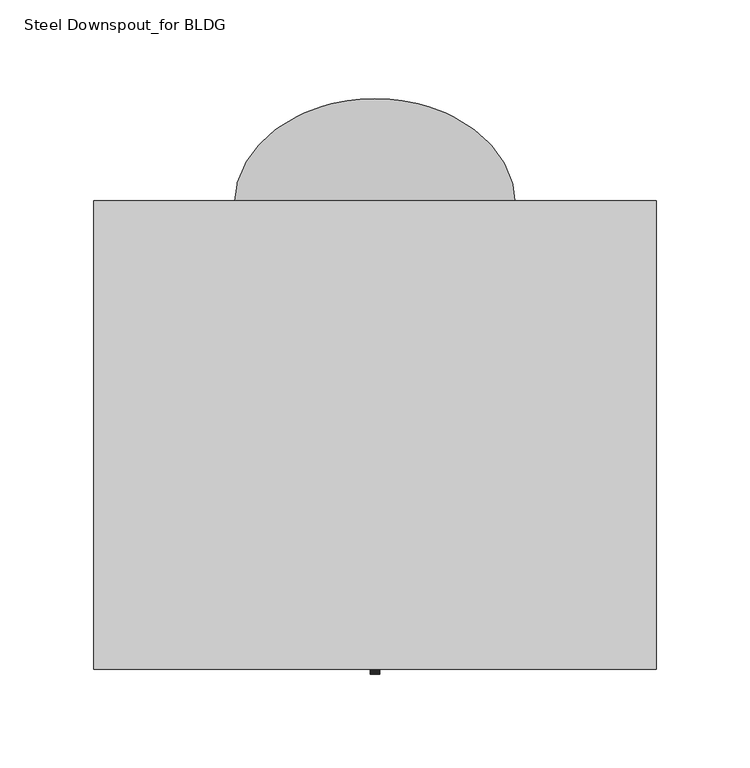
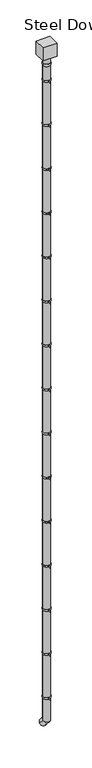
"""IFC4 building model written with IfcOpenShell, lengths in millimetres: proxy geometry, Steel Downspout_for BLDG : H_GM_AR_B07_Steel Downspout_D150."""

from ifc_helpers import new_model, si_unit, point, frame, origin, origin_with_axes, origin_2d, place, context, project, spatial, polyline, circle_curve, ellipse_curve, trimmed, segment, composite_curve, outline, extrude, source, transform, mapped, element, save
from ifc_brep_helpers import plane_surface, cylinder_surface, revolved_surface, advanced_brep


def steel_downspout_for_bldg_2e53916e(model_context):
    return source(origin(), model_context, "Body", "SolidModel", [
        extrude(outline(polyline([(2.5, -125.0), (-2.5, -125.0), (-2.5, -50.0), (2.5, -50.0), (2.5, -125.0)])), frame((0.0, 0.0, -556.0), z_axis=(0.0, 0.0, 1.0), x_axis=(1.0, 0.0, 0.0)), (0.0, 0.0, 1.0), 32.0),
        extrude(outline(composite_curve([segment(trimmed(circle_curve(origin_2d(), 80.0), [point((0.0, 80.0))], [point((0.0, -80.0))], False, "CARTESIAN"), True, "CONTINUOUS"), segment(trimmed(circle_curve(origin_2d(), 80.0), [point((0.0, -80.0))], [point((0.0, 80.0))], False, "CARTESIAN"), True, "CONTINUOUS")], self_intersect=False), holes=[composite_curve([segment(trimmed(circle_curve(origin_2d(), 75.0), [point((0.0, 75.0))], [point((0.0, -75.0))], True, "CARTESIAN"), True, "CONTINUOUS"), segment(trimmed(circle_curve(origin_2d(), 75.0), [point((0.0, -75.0))], [point((0.0, 75.0))], True, "CARTESIAN"), True, "CONTINUOUS")], self_intersect=False)]), frame((0.0, 0.0, -556.0), z_axis=(0.0, 0.0, 1.0), x_axis=(1.0, 0.0, 0.0)), (0.0, 0.0, 1.0), 32.0),
        extrude(outline(polyline([(2.5, -125.0), (-2.5, -125.0), (-2.5, -50.0), (2.5, -50.0), (2.5, -125.0)])), frame((0.0, 0.0, -1556.0), z_axis=(0.0, 0.0, 1.0), x_axis=(1.0, 0.0, 0.0)), (0.0, 0.0, 1.0), 32.0),
        extrude(outline(composite_curve([segment(trimmed(circle_curve(origin_2d(), 80.0), [point((0.0, 80.0))], [point((0.0, -80.0))], False, "CARTESIAN"), True, "CONTINUOUS"), segment(trimmed(circle_curve(origin_2d(), 80.0), [point((0.0, -80.0))], [point((0.0, 80.0))], False, "CARTESIAN"), True, "CONTINUOUS")], self_intersect=False), holes=[composite_curve([segment(trimmed(circle_curve(origin_2d(), 75.0), [point((0.0, 75.0))], [point((0.0, -75.0))], True, "CARTESIAN"), True, "CONTINUOUS"), segment(trimmed(circle_curve(origin_2d(), 75.0), [point((0.0, -75.0))], [point((0.0, 75.0))], True, "CARTESIAN"), True, "CONTINUOUS")], self_intersect=False)]), frame((0.0, 0.0, -1556.0), z_axis=(0.0, 0.0, 1.0), x_axis=(1.0, 0.0, 0.0)), (0.0, 0.0, 1.0), 32.0),
        extrude(outline(polyline([(2.5, -125.0), (-2.5, -125.0), (-2.5, -50.0), (2.5, -50.0), (2.5, -125.0)])), frame((0.0, 0.0, -2556.0), z_axis=(0.0, 0.0, 1.0), x_axis=(1.0, 0.0, 0.0)), (0.0, 0.0, 1.0), 32.0),
        extrude(outline(composite_curve([segment(trimmed(circle_curve(origin_2d(), 80.0), [point((0.0, 80.0))], [point((0.0, -80.0))], False, "CARTESIAN"), True, "CONTINUOUS"), segment(trimmed(circle_curve(origin_2d(), 80.0), [point((0.0, -80.0))], [point((0.0, 80.0))], False, "CARTESIAN"), True, "CONTINUOUS")], self_intersect=False), holes=[composite_curve([segment(trimmed(circle_curve(origin_2d(), 75.0), [point((0.0, 75.0))], [point((0.0, -75.0))], True, "CARTESIAN"), True, "CONTINUOUS"), segment(trimmed(circle_curve(origin_2d(), 75.0), [point((0.0, -75.0))], [point((0.0, 75.0))], True, "CARTESIAN"), True, "CONTINUOUS")], self_intersect=False)]), frame((0.0, 0.0, -2556.0), z_axis=(0.0, 0.0, 1.0), x_axis=(1.0, 0.0, 0.0)), (0.0, 0.0, 1.0), 32.0),
        extrude(outline(polyline([(2.5, -125.0), (-2.5, -125.0), (-2.5, -50.0), (2.5, -50.0), (2.5, -125.0)])), frame((0.0, 0.0, -3556.0), z_axis=(0.0, 0.0, 1.0), x_axis=(1.0, 0.0, 0.0)), (0.0, 0.0, 1.0), 32.0),
        extrude(outline(composite_curve([segment(trimmed(circle_curve(origin_2d(), 80.0), [point((0.0, 80.0))], [point((0.0, -80.0))], False, "CARTESIAN"), True, "CONTINUOUS"), segment(trimmed(circle_curve(origin_2d(), 80.0), [point((0.0, -80.0))], [point((0.0, 80.0))], False, "CARTESIAN"), True, "CONTINUOUS")], self_intersect=False), holes=[composite_curve([segment(trimmed(circle_curve(origin_2d(), 75.0), [point((0.0, 75.0))], [point((0.0, -75.0))], True, "CARTESIAN"), True, "CONTINUOUS"), segment(trimmed(circle_curve(origin_2d(), 75.0), [point((0.0, -75.0))], [point((0.0, 75.0))], True, "CARTESIAN"), True, "CONTINUOUS")], self_intersect=False)]), frame((0.0, 0.0, -3556.0), z_axis=(0.0, 0.0, 1.0), x_axis=(1.0, 0.0, 0.0)), (0.0, 0.0, 1.0), 32.0),
        extrude(outline(polyline([(2.5, -125.0), (-2.5, -125.0), (-2.5, -50.0), (2.5, -50.0), (2.5, -125.0)])), frame((0.0, 0.0, -4556.0), z_axis=(0.0, 0.0, 1.0), x_axis=(1.0, 0.0, 0.0)), (0.0, 0.0, 1.0), 32.0),
        extrude(outline(composite_curve([segment(trimmed(circle_curve(origin_2d(), 80.0), [point((0.0, 80.0))], [point((0.0, -80.0))], False, "CARTESIAN"), True, "CONTINUOUS"), segment(trimmed(circle_curve(origin_2d(), 80.0), [point((0.0, -80.0))], [point((0.0, 80.0))], False, "CARTESIAN"), True, "CONTINUOUS")], self_intersect=False), holes=[composite_curve([segment(trimmed(circle_curve(origin_2d(), 75.0), [point((0.0, 75.0))], [point((0.0, -75.0))], True, "CARTESIAN"), True, "CONTINUOUS"), segment(trimmed(circle_curve(origin_2d(), 75.0), [point((0.0, -75.0))], [point((0.0, 75.0))], True, "CARTESIAN"), True, "CONTINUOUS")], self_intersect=False)]), frame((0.0, 0.0, -4556.0), z_axis=(0.0, 0.0, 1.0), x_axis=(1.0, 0.0, 0.0)), (0.0, 0.0, 1.0), 32.0),
        extrude(outline(polyline([(2.5, -125.0), (-2.5, -125.0), (-2.5, -50.0), (2.5, -50.0), (2.5, -125.0)])), frame((0.0, 0.0, -5556.0), z_axis=(0.0, 0.0, 1.0), x_axis=(1.0, 0.0, 0.0)), (0.0, 0.0, 1.0), 32.0),
        extrude(outline(composite_curve([segment(trimmed(circle_curve(origin_2d(), 80.0), [point((0.0, 80.0))], [point((0.0, -80.0))], False, "CARTESIAN"), True, "CONTINUOUS"), segment(trimmed(circle_curve(origin_2d(), 80.0), [point((0.0, -80.0))], [point((0.0, 80.0))], False, "CARTESIAN"), True, "CONTINUOUS")], self_intersect=False), holes=[composite_curve([segment(trimmed(circle_curve(origin_2d(), 75.0), [point((0.0, 75.0))], [point((0.0, -75.0))], True, "CARTESIAN"), True, "CONTINUOUS"), segment(trimmed(circle_curve(origin_2d(), 75.0), [point((0.0, -75.0))], [point((0.0, 75.0))], True, "CARTESIAN"), True, "CONTINUOUS")], self_intersect=False)]), frame((0.0, 0.0, -5556.0), z_axis=(0.0, 0.0, 1.0), x_axis=(1.0, 0.0, 0.0)), (0.0, 0.0, 1.0), 32.0),
        extrude(outline(polyline([(2.5, -125.0), (-2.5, -125.0), (-2.5, -50.0), (2.5, -50.0), (2.5, -125.0)])), frame((0.0, 0.0, -6556.0), z_axis=(0.0, 0.0, 1.0), x_axis=(1.0, 0.0, 0.0)), (0.0, 0.0, 1.0), 32.0),
        extrude(outline(composite_curve([segment(trimmed(circle_curve(origin_2d(), 80.0), [point((0.0, 80.0))], [point((0.0, -80.0))], False, "CARTESIAN"), True, "CONTINUOUS"), segment(trimmed(circle_curve(origin_2d(), 80.0), [point((0.0, -80.0))], [point((0.0, 80.0))], False, "CARTESIAN"), True, "CONTINUOUS")], self_intersect=False), holes=[composite_curve([segment(trimmed(circle_curve(origin_2d(), 75.0), [point((0.0, 75.0))], [point((0.0, -75.0))], True, "CARTESIAN"), True, "CONTINUOUS"), segment(trimmed(circle_curve(origin_2d(), 75.0), [point((0.0, -75.0))], [point((0.0, 75.0))], True, "CARTESIAN"), True, "CONTINUOUS")], self_intersect=False)]), frame((0.0, 0.0, -6556.0), z_axis=(0.0, 0.0, 1.0), x_axis=(1.0, 0.0, 0.0)), (0.0, 0.0, 1.0), 32.0),
        extrude(outline(polyline([(2.5, -125.0), (-2.5, -125.0), (-2.5, -50.0), (2.5, -50.0), (2.5, -125.0)])), frame((0.0, 0.0, -7556.0), z_axis=(0.0, 0.0, 1.0), x_axis=(1.0, 0.0, 0.0)), (0.0, 0.0, 1.0), 32.0),
        extrude(outline(composite_curve([segment(trimmed(circle_curve(origin_2d(), 80.0), [point((0.0, 80.0))], [point((0.0, -80.0))], False, "CARTESIAN"), True, "CONTINUOUS"), segment(trimmed(circle_curve(origin_2d(), 80.0), [point((0.0, -80.0))], [point((0.0, 80.0))], False, "CARTESIAN"), True, "CONTINUOUS")], self_intersect=False), holes=[composite_curve([segment(trimmed(circle_curve(origin_2d(), 75.0), [point((0.0, 75.0))], [point((0.0, -75.0))], True, "CARTESIAN"), True, "CONTINUOUS"), segment(trimmed(circle_curve(origin_2d(), 75.0), [point((0.0, -75.0))], [point((0.0, 75.0))], True, "CARTESIAN"), True, "CONTINUOUS")], self_intersect=False)]), frame((0.0, 0.0, -7556.0), z_axis=(0.0, 0.0, 1.0), x_axis=(1.0, 0.0, 0.0)), (0.0, 0.0, 1.0), 32.0),
        extrude(outline(polyline([(2.5, -125.0), (-2.5, -125.0), (-2.5, -50.0), (2.5, -50.0), (2.5, -125.0)])), frame((0.0, 0.0, -8556.0), z_axis=(0.0, 0.0, 1.0), x_axis=(1.0, 0.0, 0.0)), (0.0, 0.0, 1.0), 32.0),
        extrude(outline(composite_curve([segment(trimmed(circle_curve(origin_2d(), 80.0), [point((0.0, 80.0))], [point((0.0, -80.0))], False, "CARTESIAN"), True, "CONTINUOUS"), segment(trimmed(circle_curve(origin_2d(), 80.0), [point((0.0, -80.0))], [point((0.0, 80.0))], False, "CARTESIAN"), True, "CONTINUOUS")], self_intersect=False), holes=[composite_curve([segment(trimmed(circle_curve(origin_2d(), 75.0), [point((0.0, 75.0))], [point((0.0, -75.0))], True, "CARTESIAN"), True, "CONTINUOUS"), segment(trimmed(circle_curve(origin_2d(), 75.0), [point((0.0, -75.0))], [point((0.0, 75.0))], True, "CARTESIAN"), True, "CONTINUOUS")], self_intersect=False)]), frame((0.0, 0.0, -8556.0), z_axis=(0.0, 0.0, 1.0), x_axis=(1.0, 0.0, 0.0)), (0.0, 0.0, 1.0), 32.0),
        extrude(outline(polyline([(2.5, -125.0), (-2.5, -125.0), (-2.5, -50.0), (2.5, -50.0), (2.5, -125.0)])), frame((0.0, 0.0, -9556.0), z_axis=(0.0, 0.0, 1.0), x_axis=(1.0, 0.0, 0.0)), (0.0, 0.0, 1.0), 32.0),
        extrude(outline(composite_curve([segment(trimmed(circle_curve(origin_2d(), 80.0), [point((0.0, 80.0))], [point((0.0, -80.0))], False, "CARTESIAN"), True, "CONTINUOUS"), segment(trimmed(circle_curve(origin_2d(), 80.0), [point((0.0, -80.0))], [point((0.0, 80.0))], False, "CARTESIAN"), True, "CONTINUOUS")], self_intersect=False), holes=[composite_curve([segment(trimmed(circle_curve(origin_2d(), 75.0), [point((0.0, 75.0))], [point((0.0, -75.0))], True, "CARTESIAN"), True, "CONTINUOUS"), segment(trimmed(circle_curve(origin_2d(), 75.0), [point((0.0, -75.0))], [point((0.0, 75.0))], True, "CARTESIAN"), True, "CONTINUOUS")], self_intersect=False)]), frame((0.0, 0.0, -9556.0), z_axis=(0.0, 0.0, 1.0), x_axis=(1.0, 0.0, 0.0)), (0.0, 0.0, 1.0), 32.0),
        extrude(outline(polyline([(2.5, -125.0), (-2.5, -125.0), (-2.5, -50.0), (2.5, -50.0), (2.5, -125.0)])), frame((0.0, 0.0, -10556.0), z_axis=(0.0, 0.0, 1.0), x_axis=(1.0, 0.0, 0.0)), (0.0, 0.0, 1.0), 32.0),
        extrude(outline(composite_curve([segment(trimmed(circle_curve(origin_2d(), 80.0), [point((0.0, 80.0))], [point((0.0, -80.0))], False, "CARTESIAN"), True, "CONTINUOUS"), segment(trimmed(circle_curve(origin_2d(), 80.0), [point((0.0, -80.0))], [point((0.0, 80.0))], False, "CARTESIAN"), True, "CONTINUOUS")], self_intersect=False), holes=[composite_curve([segment(trimmed(circle_curve(origin_2d(), 75.0), [point((0.0, 75.0))], [point((0.0, -75.0))], True, "CARTESIAN"), True, "CONTINUOUS"), segment(trimmed(circle_curve(origin_2d(), 75.0), [point((0.0, -75.0))], [point((0.0, 75.0))], True, "CARTESIAN"), True, "CONTINUOUS")], self_intersect=False)]), frame((0.0, 0.0, -10556.0), z_axis=(0.0, 0.0, 1.0), x_axis=(1.0, 0.0, 0.0)), (0.0, 0.0, 1.0), 32.0),
        extrude(outline(polyline([(2.5, -125.0), (-2.5, -125.0), (-2.5, -50.0), (2.5, -50.0), (2.5, -125.0)])), frame((0.0, 0.0, -11556.0), z_axis=(0.0, 0.0, 1.0), x_axis=(1.0, 0.0, 0.0)), (0.0, 0.0, 1.0), 32.0),
        extrude(outline(composite_curve([segment(trimmed(circle_curve(origin_2d(), 80.0), [point((0.0, 80.0))], [point((0.0, -80.0))], False, "CARTESIAN"), True, "CONTINUOUS"), segment(trimmed(circle_curve(origin_2d(), 80.0), [point((0.0, -80.0))], [point((0.0, 80.0))], False, "CARTESIAN"), True, "CONTINUOUS")], self_intersect=False), holes=[composite_curve([segment(trimmed(circle_curve(origin_2d(), 75.0), [point((0.0, 75.0))], [point((0.0, -75.0))], True, "CARTESIAN"), True, "CONTINUOUS"), segment(trimmed(circle_curve(origin_2d(), 75.0), [point((0.0, -75.0))], [point((0.0, 75.0))], True, "CARTESIAN"), True, "CONTINUOUS")], self_intersect=False)]), frame((0.0, 0.0, -11556.0), z_axis=(0.0, 0.0, 1.0), x_axis=(1.0, 0.0, 0.0)), (0.0, 0.0, 1.0), 32.0),
        extrude(outline(polyline([(2.5, -125.0), (-2.5, -125.0), (-2.5, -50.0), (2.5, -50.0), (2.5, -125.0)])), frame((0.0, 0.0, -12556.0), z_axis=(0.0, 0.0, 1.0), x_axis=(1.0, 0.0, 0.0)), (0.0, 0.0, 1.0), 32.0),
        extrude(outline(composite_curve([segment(trimmed(circle_curve(origin_2d(), 80.0), [point((0.0, 80.0))], [point((0.0, -80.0))], False, "CARTESIAN"), True, "CONTINUOUS"), segment(trimmed(circle_curve(origin_2d(), 80.0), [point((0.0, -80.0))], [point((0.0, 80.0))], False, "CARTESIAN"), True, "CONTINUOUS")], self_intersect=False), holes=[composite_curve([segment(trimmed(circle_curve(origin_2d(), 75.0), [point((0.0, 75.0))], [point((0.0, -75.0))], True, "CARTESIAN"), True, "CONTINUOUS"), segment(trimmed(circle_curve(origin_2d(), 75.0), [point((0.0, -75.0))], [point((0.0, 75.0))], True, "CARTESIAN"), True, "CONTINUOUS")], self_intersect=False)]), frame((0.0, 0.0, -12556.0), z_axis=(0.0, 0.0, 1.0), x_axis=(1.0, 0.0, 0.0)), (0.0, 0.0, 1.0), 32.0),
        extrude(outline(polyline([(2.5, -125.0), (-2.5, -125.0), (-2.5, -50.0), (2.5, -50.0), (2.5, -125.0)])), frame((0.0, 0.0, -13556.0), z_axis=(0.0, 0.0, 1.0), x_axis=(1.0, 0.0, 0.0)), (0.0, 0.0, 1.0), 32.0),
        extrude(outline(composite_curve([segment(trimmed(circle_curve(origin_2d(), 80.0), [point((0.0, 80.0))], [point((0.0, -80.0))], False, "CARTESIAN"), True, "CONTINUOUS"), segment(trimmed(circle_curve(origin_2d(), 80.0), [point((0.0, -80.0))], [point((0.0, 80.0))], False, "CARTESIAN"), True, "CONTINUOUS")], self_intersect=False), holes=[composite_curve([segment(trimmed(circle_curve(origin_2d(), 75.0), [point((0.0, 75.0))], [point((0.0, -75.0))], True, "CARTESIAN"), True, "CONTINUOUS"), segment(trimmed(circle_curve(origin_2d(), 75.0), [point((0.0, -75.0))], [point((0.0, 75.0))], True, "CARTESIAN"), True, "CONTINUOUS")], self_intersect=False)]), frame((0.0, 0.0, -13556.0), z_axis=(0.0, 0.0, 1.0), x_axis=(1.0, 0.0, 0.0)), (0.0, 0.0, 1.0), 32.0),
        advanced_brep(
        [(-75.0, 0.0, -200.0), (75.0, 0.0, -200.0), (-65.0, 0.0, -200.0), (65.0, 0.0, -200.0), (-65.0, 0.0, -15056.0), (65.0, 0.0, -15056.0), (-75.0, 0.0, -15056.0), (75.0, 0.0, -15056.0), (-75.0, 125.386264, -15200.2403969), (75.0, 125.386264, -15200.2403969), (-65.0, 125.386264, -15200.2403969), (65.0, 125.386264, -15200.2403969)],
        [
            (0, 1, circle_curve(frame((0.0, 0.0, -200.0), z_axis=(0.0, 0.0, 1.0), x_axis=(1.0, 0.0, 0.0)), 75.0)),
            (1, 0, circle_curve(frame((0.0, 0.0, -200.0), z_axis=(0.0, 0.0, 1.0), x_axis=(1.0, 0.0, 0.0)), 75.0)),
            (2, 3, circle_curve(frame((0.0, 0.0, -200.0), z_axis=(0.0, 0.0, -1.0), x_axis=(1.0, 0.0, 0.0)), 65.0)),
            (3, 2, circle_curve(frame((0.0, 0.0, -200.0), z_axis=(0.0, 0.0, -1.0), x_axis=(1.0, 0.0, 0.0)), 65.0)),
            (2, 4),
            (4, 5, ellipse_curve(frame((0.0, 0.0, -15056.0), z_axis=(0.0, 0.3502073812593857, -0.9366721892484282), x_axis=(0.0, -0.9366721892484282, -0.35020738125938544)), 69.3946086, 65.0)),
            (5, 3),
            (5, 4, ellipse_curve(frame((0.0, 0.0, -15056.0), z_axis=(0.0, 0.3502073812593857, -0.9366721892484282), x_axis=(0.0, -0.9366721892484282, -0.35020738125938544)), 69.3946086, 65.0)),
            (0, 6),
            (6, 7, ellipse_curve(frame((0.0, 0.0, -15056.0), z_axis=(0.0, -0.3502073812593857, 0.9366721892484282), x_axis=(0.0, 0.9366721892484282, 0.35020738125938544)), 80.0707023, 75.0)),
            (7, 1),
            (7, 6, ellipse_curve(frame((0.0, 0.0, -15056.0), z_axis=(0.0, -0.3502073812593857, 0.9366721892484282), x_axis=(0.0, 0.9366721892484282, 0.35020738125938544)), 80.0707023, 75.0)),
            (8, 9, circle_curve(frame((0.0, 125.386264, -15200.2403969), z_axis=(0.0, 0.6560590289903756, -0.7547095802228865), x_axis=(1.0, 0.0, 0.0)), 75.0)),
            (9, 8, circle_curve(frame((0.0, 125.386264, -15200.2403969), z_axis=(0.0, 0.6560590289903756, -0.7547095802228865), x_axis=(1.0, 0.0, 0.0)), 75.0)),
            (10, 11, circle_curve(frame((0.0, 125.386264, -15200.2403969), z_axis=(0.0, -0.6560590289903756, 0.7547095802228865), x_axis=(1.0, 0.0, 0.0)), 65.0)),
            (11, 10, circle_curve(frame((0.0, 125.386264, -15200.2403969), z_axis=(0.0, -0.6560590289903756, 0.7547095802228865), x_axis=(1.0, 0.0, 0.0)), 65.0)),
            (4, 10),
            (11, 5),
            (6, 8),
            (9, 7),
        ],
        [
            plane_surface(frame((0.0, 0.0, -200.0), z_axis=(0.0, 0.0, 1.0), x_axis=(1.0, 0.0, 0.0))),
            revolved_surface(polyline([(65.0, 0.0, -15080.302504151327), (65.0, 0.0, -200.0)]), (0.0, 0.0, -200.0), (0.0, 0.0, -1.0)),
            cylinder_surface(frame((0.0, 0.0, -200.0), z_axis=(0.0, 0.0, 1.0), x_axis=(1.0, 0.0, 0.0)), 75.0),
            plane_surface(frame((0.0, 125.386264, -15200.2403969), z_axis=(0.0, 0.6560590289903756, -0.7547095802228865), x_axis=(1.0, 0.0, 0.0))),
            revolved_surface(polyline([(65.0, 125.38626404697672, -15200.240396859164), (65.0, -15.94387727555355, -15037.658667293588)]), (0.0, 0.0, -15056.0), (0.0, 0.6560590289903756, -0.7547095802228865)),
            cylinder_surface(frame((0.0, 0.0, -15056.0), z_axis=(0.0, -0.6560590289903756, 0.7547095802228865), x_axis=(1.0, 0.0, 0.0)), 75.0),
        ],
        [
            (0, [[1, 2], [3, 4]]),
            (1, [[-3, 5, 6, 7]]),
            (1, [[-4, -7, 8, -5]]),
            (2, [[-1, 9, 10, 11]]),
            (2, [[-2, -11, 12, -9]]),
            (3, [[13, 14], [15, 16]]),
            (4, [[-6, 17, -16, 18]]),
            (4, [[-8, -18, -15, -17]]),
            (5, [[-10, 19, -14, 20]]),
            (5, [[-12, -20, -13, -19]]),
        ],
    ),
        extrude(outline(polyline([(150.0, 125.0), (150.0, -125.0), (-150.0, -125.0), (-150.0, 125.0), (150.0, 125.0)])), origin_with_axes(), (0.0, 0.0, 1.0), 300.0),
        extrude(outline(polyline([(2.5, -125.0), (-2.5, -125.0), (-2.5, -50.0), (2.5, -50.0), (2.5, -125.0)])), frame((0.0, 0.0, -14556.0), z_axis=(0.0, 0.0, 1.0), x_axis=(1.0, 0.0, 0.0)), (0.0, 0.0, 1.0), 32.0),
        extrude(outline(composite_curve([segment(trimmed(circle_curve(origin_2d(), 80.0), [point((0.0, 80.0))], [point((0.0, -80.0))], False, "CARTESIAN"), True, "CONTINUOUS"), segment(trimmed(circle_curve(origin_2d(), 80.0), [point((0.0, -80.0))], [point((0.0, 80.0))], False, "CARTESIAN"), True, "CONTINUOUS")], self_intersect=False), holes=[composite_curve([segment(trimmed(circle_curve(origin_2d(), 75.0), [point((0.0, 75.0))], [point((0.0, -75.0))], True, "CARTESIAN"), True, "CONTINUOUS"), segment(trimmed(circle_curve(origin_2d(), 75.0), [point((0.0, -75.0))], [point((0.0, 75.0))], True, "CARTESIAN"), True, "CONTINUOUS")], self_intersect=False)]), frame((0.0, 0.0, -14556.0), z_axis=(0.0, 0.0, 1.0), x_axis=(1.0, 0.0, 0.0)), (0.0, 0.0, 1.0), 32.0),
        extrude(outline(composite_curve([segment(trimmed(circle_curve(origin_2d(), 80.0), [point((-80.0, 0.0))], [point((80.0, 0.0))], False, "CARTESIAN"), True, "CONTINUOUS"), segment(trimmed(circle_curve(origin_2d(), 80.0), [point((80.0, 0.0))], [point((-80.0, 0.0))], False, "CARTESIAN"), True, "CONTINUOUS")], self_intersect=False), holes=[composite_curve([segment(trimmed(circle_curve(origin_2d(), 65.0), [point((-65.0, 0.0))], [point((65.0, 0.0))], True, "CARTESIAN"), True, "CONTINUOUS"), segment(trimmed(circle_curve(origin_2d(), 65.0), [point((65.0, 0.0))], [point((-65.0, 0.0))], True, "CARTESIAN"), True, "CONTINUOUS")], self_intersect=False)]), frame((0.0, 0.0, -200.0), z_axis=(0.0, 0.0, 1.0), x_axis=(1.0, 0.0, 0.0)), (0.0, 0.0, 1.0), 50.0),
        extrude(outline(composite_curve([segment(trimmed(circle_curve(origin_2d(), 75.0), [point((-75.0, 0.0))], [point((75.0, 0.0))], False, "CARTESIAN"), True, "CONTINUOUS"), segment(trimmed(circle_curve(origin_2d(), 75.0), [point((75.0, 0.0))], [point((-75.0, 0.0))], False, "CARTESIAN"), True, "CONTINUOUS")], self_intersect=False), holes=[composite_curve([segment(trimmed(circle_curve(origin_2d(), 65.0), [point((-65.0, 0.0))], [point((65.0, 0.0))], True, "CARTESIAN"), True, "CONTINUOUS"), segment(trimmed(circle_curve(origin_2d(), 65.0), [point((65.0, 0.0))], [point((-65.0, 0.0))], True, "CARTESIAN"), True, "CONTINUOUS")], self_intersect=False)]), frame((0.0, 0.0, -150.0), z_axis=(0.0, 0.0, 1.0), x_axis=(1.0, 0.0, 0.0)), (0.0, 0.0, 1.0), 150.0),
    ])


if __name__ == "__main__":
    model = new_model("IFC4")
    model_context = context("Model", 3, world=origin())
    ifc_project = project(units=[si_unit("LENGTHUNIT", "METRE", prefix="MILLI")], contexts=[model_context])
    site = spatial("IfcSite", under=ifc_project)
    building = spatial("IfcBuilding", under=site)
    placement = place(None, origin())
    steel_downspout_for_bldg_shape = steel_downspout_for_bldg_2e53916e(model_context)
    element("IfcBuildingElementProxy", 1, Name="Steel Downspout_for BLDG : H_GM_AR_B07_Steel Downspout_D150", ObjectType="Steel Downspout_for BLDG : H_GM_AR_B07_Steel Downspout_D150", at=placement, inside=building, context=model_context, shape_type="MappedRepresentation", body=[
        mapped(steel_downspout_for_bldg_shape, transform((0.0, 0.0, 0.0), x_axis=(1.0, 0.0, 0.0), y_axis=(0.0, 1.0, 0.0), z_axis=(0.0, 0.0, 1.0))),
    ])
    save(model, "model.ifc")

# Revit data of these elements
# Type "Steel Downspout_for BLDG : H_GM_AR_B07_Steel Downspout_D150"
#   외벽 거리 = 100 mm
#   Rainwater Downpipe Height [instance default] = 15056 mm
#   H [instance default] = 15056 mm
#   r_int. = 65 mm
#   r_bold = 80 mm
#   r = 75 mm
#   D = 150 mm
#   Box Width = 300 mm
#   Box Length = 250 mm
#   Box Height = 300 mm
#   EA [instance default] = 15
#   Material_Name = 00_Metal_Steel
#   Default Elevation = 0
# Element 1 (IfcBuildingElementProxy, "Steel Downspout_for BLDG : H_GM_AR_B07_Steel Downspout_D150")
#   Materials on its faces: "00_Metal_Steel"
# Materials
#   "00_Metal_Steel": class "Metal", colour RGB 148 148 148, transparency 0, Description = "Steel", Cost = 0, Image = Doors - Windows.Glazed Curtain Walls.Stainless Steel Curtain Wall.jpg
